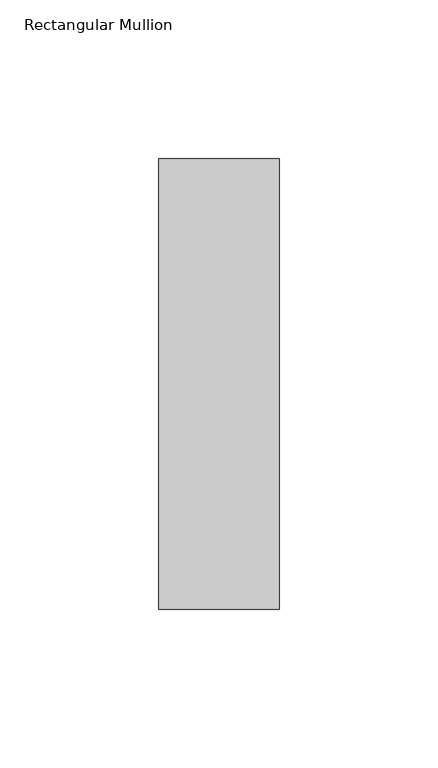
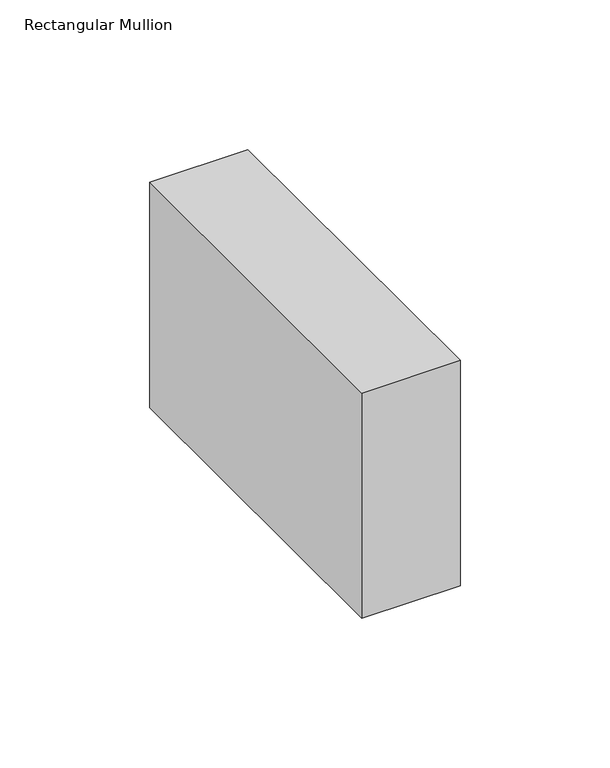
"""IFC4 building model written with IfcOpenShell, lengths in millimetres: member geometry, Rectangular Mullion : NLRS_21_CWM_hsb-regel 38x142_gen_rsf."""

from ifc_helpers import new_model, si_unit, frame, origin, place, context, project, spatial, polyline, outline, extrude, source, transform, mapped, element, save


def rectangular_mullion_0457e6f6(model_context):
    return source(origin(), model_context, "Body", "SweptSolid", [
        extrude(outline(polyline([(19.0, -71.0), (-19.0, -71.0), (-19.0, 71.0), (19.0, 71.0), (19.0, -71.0)])), frame((0.0, 0.0, -92.0), z_axis=(0.0, 0.0, 1.0), x_axis=(1.0, 0.0, 0.0)), (0.0, 0.0, 1.0), 92.0),
    ])


if __name__ == "__main__":
    model = new_model("IFC4")
    model_context = context("Model", 3, world=origin())
    ifc_project = project(units=[si_unit("LENGTHUNIT", "METRE", prefix="MILLI")], contexts=[model_context])
    site = spatial("IfcSite", under=ifc_project)
    building = spatial("IfcBuilding", under=site)
    placement = place(None, origin())
    rectangular_mullion_shape = rectangular_mullion_0457e6f6(model_context)
    element("IfcMember", 1, ObjectType="Rectangular Mullion : NLRS_21_CWM_hsb-regel 38x142_gen_rsf", at=placement, inside=building, context=model_context, shape_type="MappedRepresentation", body=[
        mapped(rectangular_mullion_shape, transform((0.0, 0.0, 0.0), x_axis=(1.0, 0.0, 0.0), y_axis=(0.0, 1.0, 0.0), z_axis=(0.0, 0.0, 1.0))),
    ])
    save(model, "model.ifc")

# Revit data of these elements
# Type "Rectangular Mullion : NLRS_21_CWM_hsb-regel 38x142_gen_rsf"
#   Export Type to IFC As = "IfcWall"
#   Type IfcGUID = "07M7mRoiH1CR8m_RSKIwpF"
#   Assembly Code = "21.10"
#   built-in parameter 1007322 = 0.465879 (stored number, unit not read)
#   built-in parameter 1007321 = 0.062336 (stored number, unit not read)
#   built-in parameter 1007320 = 0.062336 (stored number, unit not read)
# Element 1 (IfcMember, "Rectangular Mullion : NLRS_21_CWM_hsb-regel 38x142_gen_rsf")
#   Materials on its faces: "NLRS_i2_hout naaldhout vuren_gen_rsf"
# Materials
#   "NLRS_i2_hout naaldhout vuren_gen_rsf": class "I - Hout", colour RGB 234 199 147, transparency 0, Keynote = "i2", Manufacturer = "Revit Standards Foundation", URL = "www.revitstandards.org", Description = "hout vuren", Cost = 0
